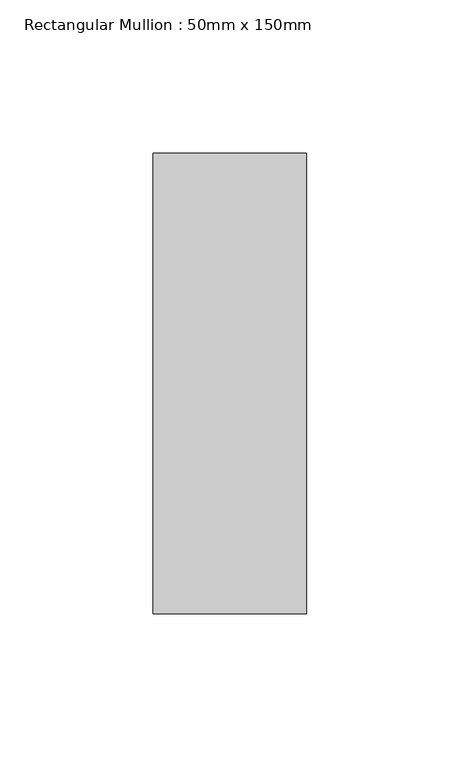
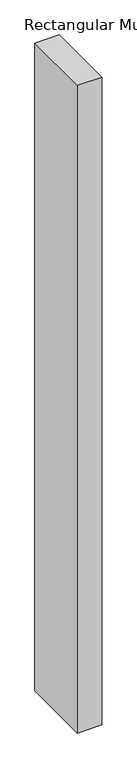
"""IFC4 building model written with IfcOpenShell, lengths in millimetres: member geometry, Rectangular Mullion : 50mm x 150mm."""

import ifcopenshell
import ifcopenshell.guid

model = None  # the IFC model being written
_history = None  # IfcOwnerHistory: only IFC2X3 demands one
_inside = {}  # id of a spatial element -> (the spatial element, [elements in it])
_under = {}  # id of a project, library or spatial element -> (it, [spatial elements below it])
_declared = {}  # id of a project -> (the project, [libraries it declares])
_typed = {}  # id of a type object -> (the type object, [elements of that type])
_made_of = {}  # id of a material, layer set ... -> (it, [elements and type objects made of it])


def new_model(schema):
    """Start an empty IFC model of exactly this schema.

    Asked for "IFC4X3", IfcOpenShell would pick the latest addendum, in which some entities
    have other attributes; the version numbers below select the first issue.
    IFC2X3 requires an IfcOwnerHistory on every rooted entity: one is made here for all.
    """
    global model, _history
    if schema == "IFC4X3":
        model = ifcopenshell.file(schema_version=(4, 3, 0, 0))
    else:
        model = ifcopenshell.file(schema=schema)
    _inside.clear()
    _under.clear()
    _declared.clear()
    _typed.clear()
    _made_of.clear()
    _history = None
    if model.schema == "IFC2X3":
        org = make("IfcOrganization", Name="unknown")
        user = make(
            "IfcPersonAndOrganization",
            ThePerson=make("IfcPerson", FamilyName="unknown"),
            TheOrganization=org,
        )
        app = make(
            "IfcApplication",
            ApplicationDeveloper=org,
            Version="unknown",
            ApplicationFullName="unknown",
            ApplicationIdentifier="unknown",
        )
        _history = make(
            "IfcOwnerHistory",
            OwningUser=user,
            OwningApplication=app,
            ChangeAction="ADDED",
            CreationDate=0,
        )
    return model


def make(cls, **values):
    """One entity of the class cls with the attributes given. An attribute that is None is left unset."""
    return model.create_entity(
        cls, **{name: value for name, value in values.items() if value is not None}
    )


def rooted(cls, **values):
    """An entity with a GlobalId (a new one), such as an element, a storey or a relation."""
    return make(cls, GlobalId=ifcopenshell.guid.new(), OwnerHistory=_history, **values)


def si_unit(unit_type, name, prefix=None):
    """IfcSIUnit, for example si_unit("LENGTHUNIT", "METRE", prefix="MILLI")."""
    return make("IfcSIUnit", UnitType=unit_type, Prefix=prefix, Name=name)


def assignment(units):
    """IfcUnitAssignment: the units of a project."""
    return None if units is None else make("IfcUnitAssignment", Units=units)


def point(xyz):
    """IfcCartesianPoint."""
    return None if xyz is None else make("IfcCartesianPoint", Coordinates=xyz)


def direction(xyz):
    """IfcDirection."""
    return None if xyz is None else make("IfcDirection", DirectionRatios=xyz)


def frame(location, z_axis=None, x_axis=None):
    """IfcAxis2Placement3D, a coordinate frame: its origin and axes. An axis left out is left unset."""
    return make(
        "IfcAxis2Placement3D",
        Location=point(location),
        Axis=direction(z_axis),
        RefDirection=direction(x_axis),
    )


def origin():
    """The frame at (0, 0, 0) with its axes left unset."""
    return frame((0.0, 0.0, 0.0))


def place(relative_to, where):
    """IfcLocalPlacement: puts the frame where relative to a parent placement (None: the world)."""
    return make(
        "IfcLocalPlacement", PlacementRelTo=relative_to, RelativePlacement=where
    )


def context(
    kind, dimensions, precision=None, world=None, true_north=None, identifier=None
):
    """IfcGeometricRepresentationContext, for example the 3D "Model" context."""
    return make(
        "IfcGeometricRepresentationContext",
        ContextIdentifier=identifier,
        ContextType=kind,
        CoordinateSpaceDimension=dimensions,
        Precision=precision,
        WorldCoordinateSystem=world,
        TrueNorth=true_north,
    )


def project(units=None, contexts=None):
    """IfcProject with its units and contexts."""
    return rooted(
        "IfcProject",
        Name="project",
        RepresentationContexts=contexts,
        UnitsInContext=assignment(units),
    )


def spatial(cls, under=None, at=None, **own):
    """A site, building, storey or space (cls), placed at a placement, below another one or the project."""
    s = rooted(cls, ObjectPlacement=at, **own)
    if under is not None:
        _under.setdefault(under.id(), (under, []))[1].append(s)
    return s


def polyline(points):
    """IfcPolyline through the points."""
    return make("IfcPolyline", Points=[point(p) for p in points])


def outline(outer, holes=None, kind="AREA"):
    """IfcArbitraryClosedProfileDef: a profile drawn as a closed curve; with holes, ...WithVoids."""
    if holes is None:
        return make("IfcArbitraryClosedProfileDef", ProfileType=kind, OuterCurve=outer)
    return make(
        "IfcArbitraryProfileDefWithVoids",
        ProfileType=kind,
        OuterCurve=outer,
        InnerCurves=holes,
    )


def extrude(swept, where, along, depth):
    """IfcExtrudedAreaSolid: the profile swept, set in the frame where, extruded along a direction by depth."""
    return make(
        "IfcExtrudedAreaSolid",
        SweptArea=swept,
        Position=where,
        ExtrudedDirection=direction(along),
        Depth=depth,
    )


def shape(context_of_items, identifier, shape_type, items):
    """IfcShapeRepresentation: the items that make up one representation, for example the "Body"."""
    return make(
        "IfcShapeRepresentation",
        ContextOfItems=context_of_items,
        RepresentationIdentifier=identifier,
        RepresentationType=shape_type,
        Items=items,
    )


def source(mapping_origin, context_of_items, identifier, shape_type, items):
    """IfcRepresentationMap: a shape defined once, which mapped items show again and again."""
    return make(
        "IfcRepresentationMap",
        MappingOrigin=mapping_origin,
        MappedRepresentation=shape(context_of_items, identifier, shape_type, items),
    )


def transform(
    local_origin,
    x_axis=None,
    y_axis=None,
    z_axis=None,
    scale=None,
    scale2=None,
    scale3=None,
    uniform=True,
):
    """IfcCartesianTransformationOperator3D, or its non-uniform kind. x_axis, y_axis, z_axis: its Axis1, 2, 3."""
    if uniform:
        return make(
            "IfcCartesianTransformationOperator3D",
            Axis1=direction(x_axis),
            Axis2=direction(y_axis),
            LocalOrigin=point(local_origin),
            Scale=scale,
            Axis3=direction(z_axis),
        )
    return make(
        "IfcCartesianTransformationOperator3DnonUniform",
        Axis1=direction(x_axis),
        Axis2=direction(y_axis),
        LocalOrigin=point(local_origin),
        Scale=scale,
        Axis3=direction(z_axis),
        Scale2=scale2,
        Scale3=scale3,
    )


def mapped(mapping_source, mapping_target):
    """IfcMappedItem: shows the shape of a source again, moved by a transform."""
    return make(
        "IfcMappedItem", MappingSource=mapping_source, MappingTarget=mapping_target
    )


def made_of(thing, what):
    """Note that an element or type object is made of a material, layer set ...; save() writes the relation."""
    if what is not None:
        _made_of.setdefault(what.id(), (what, []))[1].append(thing)
    return thing


def element(
    cls,
    number,
    at=None,
    inside=None,
    cuts=None,
    type_object=None,
    material=None,
    context=None,
    identifier="Body",
    shape_type=None,
    held_by="IfcProductDefinitionShape",
    body=None,
    shapes=None,
    **own,
):
    """One element of the class cls, such as IfcWall. Its Tag is "e" and its number.

    at: its placement. inside: the storey or other place that contains it. cuts: it is an
    opening in that element (IfcRelVoidsElement). A single representation is given by context,
    identifier, shape_type and body (its items); several are given by shapes. held_by: the class
    of the entity that holds the representations. save() writes the other relations.
    """
    e = rooted(cls, Tag="e%d" % number, ObjectPlacement=at, **own)
    if body is not None:
        shapes = [shape(context, identifier, shape_type, body)]
    if shapes is not None:
        e.Representation = make(held_by, Representations=shapes)
    if inside is not None:
        _inside.setdefault(inside.id(), (inside, []))[1].append(e)
    if cuts is not None:
        rooted(
            "IfcRelVoidsElement", RelatingBuildingElement=cuts, RelatedOpeningElement=e
        )
    if type_object is not None:
        _typed.setdefault(type_object.id(), (type_object, []))[1].append(e)
    return made_of(e, material)


def aggregate(whole, parts):
    """IfcRelAggregates: a whole, such as a stair, and the parts it consists of."""
    return rooted("IfcRelAggregates", RelatingObject=whole, RelatedObjects=parts)


def save(model, path):
    """Write the relations noted so far, then the file.

    IfcRelAggregates (storeys below a building ...), IfcRelContainedInSpatialStructure (elements
    in a storey), IfcRelDefinesByType, IfcRelAssociatesMaterial and IfcRelDeclares: one each for
    every whole, place, type object, material and project.
    """
    for whole, parts in _under.values():
        aggregate(whole, parts)
    for where, things in _inside.values():
        rooted(
            "IfcRelContainedInSpatialStructure",
            RelatedElements=things,
            RelatingStructure=where,
        )
    for kind, things in _typed.values():
        rooted("IfcRelDefinesByType", RelatedObjects=things, RelatingType=kind)
    for what, things in _made_of.values():
        rooted("IfcRelAssociatesMaterial", RelatedObjects=things, RelatingMaterial=what)
    for by, libraries in _declared.values():
        rooted("IfcRelDeclares", RelatingContext=by, RelatedDefinitions=libraries)
    model.write(path)


def rectangular_mullion_50mm_x_150mm_efa02866(model_context):
    return source(origin(), model_context, "Body", "SweptSolid", [
        extrude(outline(polyline([(0.0, 75.0), (0.0, -75.0), (-50.0, -75.0), (-50.0, 75.0), (0.0, 75.0)])), frame((0.0, 0.0, -1399.9999997), z_axis=(0.0, 0.0, 1.0), x_axis=(1.0, 0.0, 0.0)), (0.0, 0.0, 1.0), 1399.9999997),
    ])


if __name__ == "__main__":
    model = new_model("IFC4")
    model_context = context("Model", 3, world=origin())
    ifc_project = project(units=[si_unit("LENGTHUNIT", "METRE", prefix="MILLI")], contexts=[model_context])
    site = spatial("IfcSite", under=ifc_project)
    building = spatial("IfcBuilding", under=site)
    placement = place(None, origin())
    rectangular_mullion_50mm_x_150mm_shape = rectangular_mullion_50mm_x_150mm_efa02866(model_context)
    element("IfcMember", 1, ObjectType="Rectangular Mullion : 50mm x 150mm", at=placement, inside=building, context=model_context, shape_type="MappedRepresentation", body=[
        mapped(rectangular_mullion_50mm_x_150mm_shape, transform((0.0, 0.0, 0.0), x_axis=(1.0, 0.0, 0.0), y_axis=(0.0, 1.0, 0.0), z_axis=(0.0, 0.0, 1.0))),
    ])
    save(model, "model.ifc")

# Revit data of these elements
# Type "Rectangular Mullion : 50mm x 150mm"
#   built-in parameter 1007304 = 0.492126 (stored number, unit not read)
#   built-in parameter 1007301 = 0.082021 (stored number, unit not read)
#   built-in parameter 1007300 = 0.082021 (stored number, unit not read)
# Element 1 (IfcMember, "Rectangular Mullion : 50mm x 150mm")
#   Materials on its faces: "Aluminum"
# Materials
#   "Aluminum": class "Metal", colour RGB 244 244 244, transparency 0, Description = "Aluminum 6061", Cost = 0
